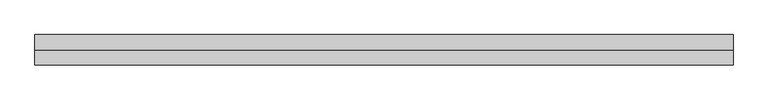
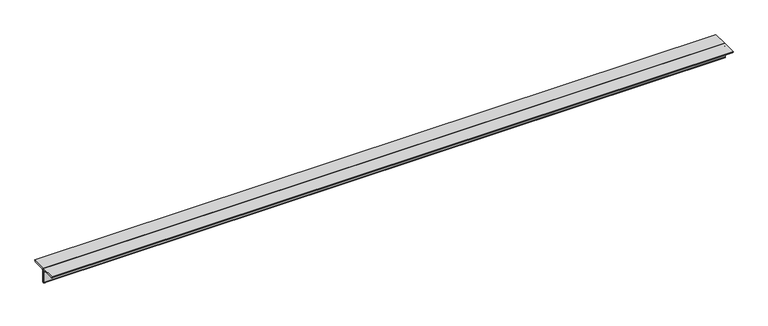
"""IFC4 building model written with IfcOpenShell, lengths in millimetres: member geometry, 0123_Steel Framing_2Ls-KSD3502 : H_SB_AR_S03_2Ls-130x130x12_HBR1."""

from ifc_helpers import new_model, si_unit, point, frame, frame_2d, origin, place, context, project, spatial, polyline, circle_curve, trimmed, segment, composite_curve, outline, extrude, source, transform, mapped, element, save


def member_72aad7bf(model_context):
    return source(origin(), model_context, "Body", "SweptSolid", [
        extrude(outline(composite_curve([segment(polyline([(0.0, 36.4), (130.0, 36.4)]), True, "CONTINUOUS"), segment(trimmed(circle_curve(frame_2d((118.0, 36.4)), 12.0), [point((130.0, 36.4))], [point((118.0, 24.4))], False, "CARTESIAN"), True, "CONTINUOUS"), segment(polyline([(118.0, 24.4), (24.0, 24.4)]), True, "CONTINUOUS"), segment(trimmed(circle_curve(frame_2d((24.0, 12.4)), 12.0), [point((24.0, 24.4))], [point((12.0, 12.4))], True, "CARTESIAN"), True, "CONTINUOUS"), segment(polyline([(12.0, 12.4), (12.0, -81.6)]), True, "CONTINUOUS"), segment(trimmed(circle_curve(frame_2d((0.0, -81.6)), 12.0), [point((12.0, -81.6))], [point((0.0, -93.6))], False, "CARTESIAN"), True, "CONTINUOUS"), segment(polyline([(0.0, -93.6), (0.0, 36.4)]), True, "CONTINUOUS")], self_intersect=False)), frame((-2991.9049386, 0.0, 0.0), z_axis=(1.0, 0.0, 0.0), x_axis=(0.0, 1.0, 0.0)), (0.0, 0.0, 1.0), 5955.4662953),
        extrude(outline(composite_curve([segment(polyline([(0.0, 36.4), (0.0, -93.6)]), True, "CONTINUOUS"), segment(trimmed(circle_curve(frame_2d((0.0, -81.6)), 12.0), [point((0.0, -93.6))], [point((-12.0, -81.6))], False, "CARTESIAN"), True, "CONTINUOUS"), segment(polyline([(-12.0, -81.6), (-12.0, 12.4)]), True, "CONTINUOUS"), segment(trimmed(circle_curve(frame_2d((-24.0, 12.4)), 12.0), [point((-12.0, 12.4))], [point((-24.0, 24.4))], True, "CARTESIAN"), True, "CONTINUOUS"), segment(polyline([(-24.0, 24.4), (-118.0, 24.4)]), True, "CONTINUOUS"), segment(trimmed(circle_curve(frame_2d((-118.0, 36.4)), 12.0), [point((-118.0, 24.4))], [point((-130.0, 36.4))], False, "CARTESIAN"), True, "CONTINUOUS"), segment(polyline([(-130.0, 36.4), (0.0, 36.4)]), True, "CONTINUOUS")], self_intersect=False)), frame((-2991.9049386, 0.0, 0.0), z_axis=(1.0, 0.0, 0.0), x_axis=(0.0, 1.0, 0.0)), (0.0, 0.0, 1.0), 5955.4662953),
    ])


if __name__ == "__main__":
    model = new_model("IFC4")
    model_context = context("Model", 3, world=origin())
    ifc_project = project(units=[si_unit("LENGTHUNIT", "METRE", prefix="MILLI")], contexts=[model_context])
    site = spatial("IfcSite", under=ifc_project)
    building = spatial("IfcBuilding", under=site)
    placement = place(None, origin())
    member_shape = member_72aad7bf(model_context)
    element("IfcMember", 1, ObjectType="0123_Steel Framing_2Ls-KSD3502 : H_SB_AR_S03_2Ls-130x130x12_HBR1", at=placement, inside=building, context=model_context, shape_type="MappedRepresentation", body=[
        mapped(member_shape, transform((0.0, 0.0, 0.0), x_axis=(1.0, 0.0, 0.0), y_axis=(0.0, 1.0, 0.0), z_axis=(0.0, 0.0, 1.0))),
    ])
    save(model, "model.ifc")

# Revit data of these elements
# Type "0123_Steel Framing_2Ls-KSD3502 : H_SB_AR_S03_2Ls-130x130x12_HBR1"
#   Type Mark = "HBR1"
#   Assembly Code = "B10"
#   Legs = "SLBB"
#   W = 8.97
#   Perimeter = 1.04 m²/m
#   Nominal Weight = 46.80 kgf/m
#   Length [instance default] = 1000 mm
#   Space = 0 mm
#   b = 130 mm
#   d = 130 mm
#   t = 12 mm
#   y = 36.4 mm
#   A = 0.005952 m²
#   Structural Material [instance default] = Steel ASTM A36
# Element 1 (IfcMember, "0123_Steel Framing_2Ls-KSD3502 : H_SB_AR_S03_2Ls-130x130x12_HBR1")
#   Materials on its faces: "Steel ASTM A36"
# Materials
#   "Steel ASTM A36": class "Metal", colour RGB 199 199 199, transparency 0, Description = "Structural steel, ASTM A36 Grade B, mill finish", Cost = 0
